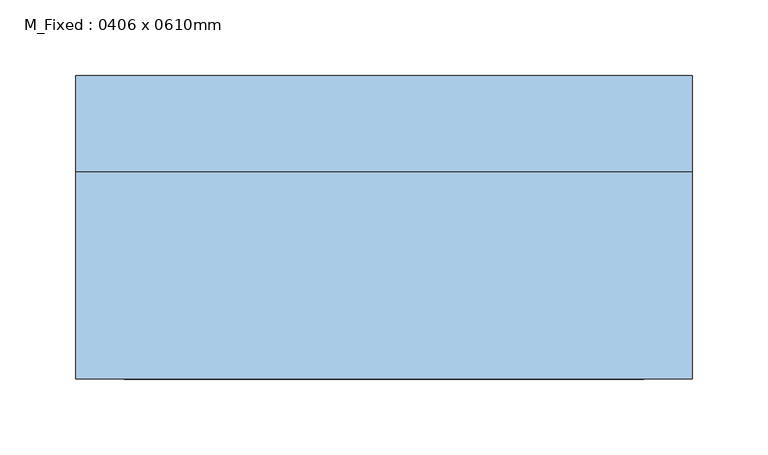
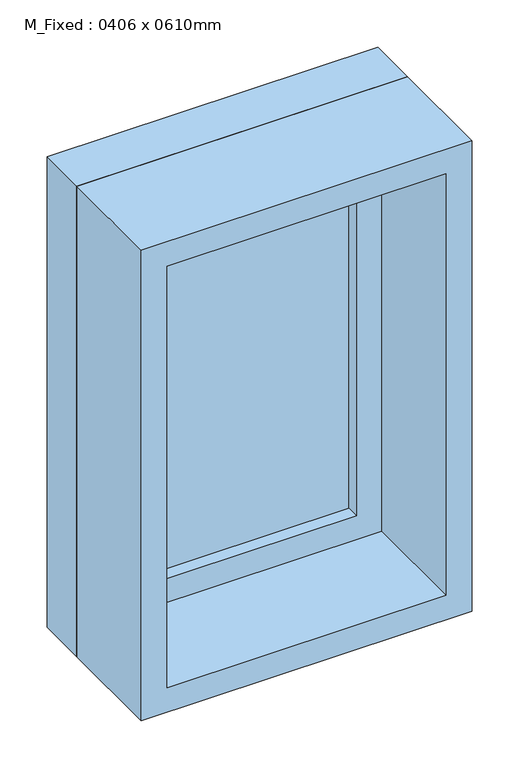
"""IFC4 building model written with IfcOpenShell, lengths in millimetres: window geometry, M_Fixed : 0406 x 0610mm."""

import ifcopenshell
import ifcopenshell.guid

model = None  # the IFC model being written
_history = None  # IfcOwnerHistory: only IFC2X3 demands one
_inside = {}  # id of a spatial element -> (the spatial element, [elements in it])
_under = {}  # id of a project, library or spatial element -> (it, [spatial elements below it])
_declared = {}  # id of a project -> (the project, [libraries it declares])
_typed = {}  # id of a type object -> (the type object, [elements of that type])
_made_of = {}  # id of a material, layer set ... -> (it, [elements and type objects made of it])


def new_model(schema):
    """Start an empty IFC model of exactly this schema.

    Asked for "IFC4X3", IfcOpenShell would pick the latest addendum, in which some entities
    have other attributes; the version numbers below select the first issue.
    IFC2X3 requires an IfcOwnerHistory on every rooted entity: one is made here for all.
    """
    global model, _history
    if schema == "IFC4X3":
        model = ifcopenshell.file(schema_version=(4, 3, 0, 0))
    else:
        model = ifcopenshell.file(schema=schema)
    _inside.clear()
    _under.clear()
    _declared.clear()
    _typed.clear()
    _made_of.clear()
    _history = None
    if model.schema == "IFC2X3":
        org = make("IfcOrganization", Name="unknown")
        user = make(
            "IfcPersonAndOrganization",
            ThePerson=make("IfcPerson", FamilyName="unknown"),
            TheOrganization=org,
        )
        app = make(
            "IfcApplication",
            ApplicationDeveloper=org,
            Version="unknown",
            ApplicationFullName="unknown",
            ApplicationIdentifier="unknown",
        )
        _history = make(
            "IfcOwnerHistory",
            OwningUser=user,
            OwningApplication=app,
            ChangeAction="ADDED",
            CreationDate=0,
        )
    return model


def make(cls, **values):
    """One entity of the class cls with the attributes given. An attribute that is None is left unset."""
    return model.create_entity(
        cls, **{name: value for name, value in values.items() if value is not None}
    )


def rooted(cls, **values):
    """An entity with a GlobalId (a new one), such as an element, a storey or a relation."""
    return make(cls, GlobalId=ifcopenshell.guid.new(), OwnerHistory=_history, **values)


def si_unit(unit_type, name, prefix=None):
    """IfcSIUnit, for example si_unit("LENGTHUNIT", "METRE", prefix="MILLI")."""
    return make("IfcSIUnit", UnitType=unit_type, Prefix=prefix, Name=name)


def assignment(units):
    """IfcUnitAssignment: the units of a project."""
    return None if units is None else make("IfcUnitAssignment", Units=units)


def point(xyz):
    """IfcCartesianPoint."""
    return None if xyz is None else make("IfcCartesianPoint", Coordinates=xyz)


def direction(xyz):
    """IfcDirection."""
    return None if xyz is None else make("IfcDirection", DirectionRatios=xyz)


def frame(location, z_axis=None, x_axis=None):
    """IfcAxis2Placement3D, a coordinate frame: its origin and axes. An axis left out is left unset."""
    return make(
        "IfcAxis2Placement3D",
        Location=point(location),
        Axis=direction(z_axis),
        RefDirection=direction(x_axis),
    )


def origin():
    """The frame at (0, 0, 0) with its axes left unset."""
    return frame((0.0, 0.0, 0.0))


def place(relative_to, where):
    """IfcLocalPlacement: puts the frame where relative to a parent placement (None: the world)."""
    return make(
        "IfcLocalPlacement", PlacementRelTo=relative_to, RelativePlacement=where
    )


def context(
    kind, dimensions, precision=None, world=None, true_north=None, identifier=None
):
    """IfcGeometricRepresentationContext, for example the 3D "Model" context."""
    return make(
        "IfcGeometricRepresentationContext",
        ContextIdentifier=identifier,
        ContextType=kind,
        CoordinateSpaceDimension=dimensions,
        Precision=precision,
        WorldCoordinateSystem=world,
        TrueNorth=true_north,
    )


def project(units=None, contexts=None):
    """IfcProject with its units and contexts."""
    return rooted(
        "IfcProject",
        Name="project",
        RepresentationContexts=contexts,
        UnitsInContext=assignment(units),
    )


def spatial(cls, under=None, at=None, **own):
    """A site, building, storey or space (cls), placed at a placement, below another one or the project."""
    s = rooted(cls, ObjectPlacement=at, **own)
    if under is not None:
        _under.setdefault(under.id(), (under, []))[1].append(s)
    return s


def polyline(points):
    """IfcPolyline through the points."""
    return make("IfcPolyline", Points=[point(p) for p in points])


def outline(outer, holes=None, kind="AREA"):
    """IfcArbitraryClosedProfileDef: a profile drawn as a closed curve; with holes, ...WithVoids."""
    if holes is None:
        return make("IfcArbitraryClosedProfileDef", ProfileType=kind, OuterCurve=outer)
    return make(
        "IfcArbitraryProfileDefWithVoids",
        ProfileType=kind,
        OuterCurve=outer,
        InnerCurves=holes,
    )


def extrude(swept, where, along, depth):
    """IfcExtrudedAreaSolid: the profile swept, set in the frame where, extruded along a direction by depth."""
    return make(
        "IfcExtrudedAreaSolid",
        SweptArea=swept,
        Position=where,
        ExtrudedDirection=direction(along),
        Depth=depth,
    )


def shape(context_of_items, identifier, shape_type, items):
    """IfcShapeRepresentation: the items that make up one representation, for example the "Body"."""
    return make(
        "IfcShapeRepresentation",
        ContextOfItems=context_of_items,
        RepresentationIdentifier=identifier,
        RepresentationType=shape_type,
        Items=items,
    )


def source(mapping_origin, context_of_items, identifier, shape_type, items):
    """IfcRepresentationMap: a shape defined once, which mapped items show again and again."""
    return make(
        "IfcRepresentationMap",
        MappingOrigin=mapping_origin,
        MappedRepresentation=shape(context_of_items, identifier, shape_type, items),
    )


def transform(
    local_origin,
    x_axis=None,
    y_axis=None,
    z_axis=None,
    scale=None,
    scale2=None,
    scale3=None,
    uniform=True,
):
    """IfcCartesianTransformationOperator3D, or its non-uniform kind. x_axis, y_axis, z_axis: its Axis1, 2, 3."""
    if uniform:
        return make(
            "IfcCartesianTransformationOperator3D",
            Axis1=direction(x_axis),
            Axis2=direction(y_axis),
            LocalOrigin=point(local_origin),
            Scale=scale,
            Axis3=direction(z_axis),
        )
    return make(
        "IfcCartesianTransformationOperator3DnonUniform",
        Axis1=direction(x_axis),
        Axis2=direction(y_axis),
        LocalOrigin=point(local_origin),
        Scale=scale,
        Axis3=direction(z_axis),
        Scale2=scale2,
        Scale3=scale3,
    )


def mapped(mapping_source, mapping_target):
    """IfcMappedItem: shows the shape of a source again, moved by a transform."""
    return make(
        "IfcMappedItem", MappingSource=mapping_source, MappingTarget=mapping_target
    )


def made_of(thing, what):
    """Note that an element or type object is made of a material, layer set ...; save() writes the relation."""
    if what is not None:
        _made_of.setdefault(what.id(), (what, []))[1].append(thing)
    return thing


def element(
    cls,
    number,
    at=None,
    inside=None,
    cuts=None,
    type_object=None,
    material=None,
    context=None,
    identifier="Body",
    shape_type=None,
    held_by="IfcProductDefinitionShape",
    body=None,
    shapes=None,
    **own,
):
    """One element of the class cls, such as IfcWall. Its Tag is "e" and its number.

    at: its placement. inside: the storey or other place that contains it. cuts: it is an
    opening in that element (IfcRelVoidsElement). A single representation is given by context,
    identifier, shape_type and body (its items); several are given by shapes. held_by: the class
    of the entity that holds the representations. save() writes the other relations.
    """
    e = rooted(cls, Tag="e%d" % number, ObjectPlacement=at, **own)
    if body is not None:
        shapes = [shape(context, identifier, shape_type, body)]
    if shapes is not None:
        e.Representation = make(held_by, Representations=shapes)
    if inside is not None:
        _inside.setdefault(inside.id(), (inside, []))[1].append(e)
    if cuts is not None:
        rooted(
            "IfcRelVoidsElement", RelatingBuildingElement=cuts, RelatedOpeningElement=e
        )
    if type_object is not None:
        _typed.setdefault(type_object.id(), (type_object, []))[1].append(e)
    return made_of(e, material)


def aggregate(whole, parts):
    """IfcRelAggregates: a whole, such as a stair, and the parts it consists of."""
    return rooted("IfcRelAggregates", RelatingObject=whole, RelatedObjects=parts)


def save(model, path):
    """Write the relations noted so far, then the file.

    IfcRelAggregates (storeys below a building ...), IfcRelContainedInSpatialStructure (elements
    in a storey), IfcRelDefinesByType, IfcRelAssociatesMaterial and IfcRelDeclares: one each for
    every whole, place, type object, material and project.
    """
    for whole, parts in _under.values():
        aggregate(whole, parts)
    for where, things in _inside.values():
        rooted(
            "IfcRelContainedInSpatialStructure",
            RelatedElements=things,
            RelatingStructure=where,
        )
    for kind, things in _typed.values():
        rooted("IfcRelDefinesByType", RelatedObjects=things, RelatingType=kind)
    for what, things in _made_of.values():
        rooted("IfcRelAssociatesMaterial", RelatedObjects=things, RelatingMaterial=what)
    for by, libraries in _declared.values():
        rooted("IfcRelDeclares", RelatingContext=by, RelatedDefinitions=libraries)
    model.write(path)


def m_fixed_0406_x_0610mm_8205b201(model_context):
    return source(origin(), model_context, "Body", "SweptSolid", [
        extrude(outline(polyline([(-140.0, 78.0), (140.0, 78.0), (140.0, 66.0), (-140.0, 66.0), (-140.0, 78.0)])), frame((0.0, 0.0, 978.0), z_axis=(0.0, 0.0, 1.0), x_axis=(1.0, 0.0, 0.0)), (0.0, 0.0, 1.0), 484.0),
        extrude(outline(polyline([(1506.0, -184.0), (934.0, -184.0), (934.0, 184.0), (1506.0, 184.0), (1506.0, -184.0)]), holes=[polyline([(1462.0, -140.0), (1462.0, 140.0), (978.0, 140.0), (978.0, -140.0), (1462.0, -140.0)])]), frame((0.0, 50.0, 0.0), z_axis=(0.0, 1.0, 0.0), x_axis=(0.0, 0.0, 1.0)), (0.0, 0.0, 1.0), 44.0),
        extrude(outline(polyline([(1525.0, -203.0), (915.0, -203.0), (915.0, 203.0), (1525.0, 203.0), (1525.0, -203.0)]), holes=[polyline([(1506.0, -184.0), (1506.0, 184.0), (934.0, 184.0), (934.0, -184.0), (1506.0, -184.0)])]), frame((0.0, 50.0, 0.0), z_axis=(0.0, 1.0, 0.0), x_axis=(0.0, 0.0, 1.0)), (0.0, 0.0, 1.0), 63.0),
        extrude(outline(polyline([(1525.0, -203.0), (915.0, -203.0), (915.0, 203.0), (1525.0, 203.0), (1525.0, -203.0)]), holes=[polyline([(1493.0, -171.0), (1493.0, 171.0), (947.0, 171.0), (947.0, -171.0), (1493.0, -171.0)])]), frame((0.0, -87.0, 0.0), z_axis=(0.0, 1.0, 0.0), x_axis=(0.0, 0.0, 1.0)), (0.0, 0.0, 1.0), 137.0),
    ])


if __name__ == "__main__":
    model = new_model("IFC4")
    model_context = context("Model", 3, world=origin())
    ifc_project = project(units=[si_unit("LENGTHUNIT", "METRE", prefix="MILLI")], contexts=[model_context])
    site = spatial("IfcSite", under=ifc_project)
    building = spatial("IfcBuilding", under=site)
    placement = place(None, origin())
    m_fixed_0406_x_0610mm_shape = m_fixed_0406_x_0610mm_8205b201(model_context)
    element("IfcWindow", 1, ObjectType="M_Fixed : 0406 x 0610mm", at=placement, inside=building, context=model_context, shape_type="MappedRepresentation", body=[
        mapped(m_fixed_0406_x_0610mm_shape, transform((0.0, 0.0, 0.0), x_axis=(1.0, 0.0, 0.0), y_axis=(0.0, 1.0, 0.0), z_axis=(0.0, 0.0, 1.0))),
    ])
    save(model, "model.ifc")

# Revit data of these elements
# Type "M_Fixed : 0406 x 0610mm"
#   Type Mark = "24"
#   Construction Type Id = "GSP4R"
#   Analytic Construction = "1/8 in Pilkington single glazing"
#   Visual Light Transmittance = 0.9
#   Thermal Resistance (R) = 0.271106 (m²·K)/W
#   Solar Heat Gain Coefficient = 0.78
#   Heat Transfer Coefficient (U) = 3.6886 W/(m²·K)
#   Height = 2' - 0.01575"
#   Default Sill Height = 3' - 0.02362"
#   Width = 1' - 3.98425"
#   Window Inset = 0' - 0.74803"
#   Frame Exterior Material = Sash
#   Frame Interior Material = Sash
#   Glass Pane Material = Glass
#   Sash = Sash
#   Wall Closure = (empty or 0)
# Element 1 (IfcWindow, "M_Fixed : 0406 x 0610mm")
#   Materials on its faces: "Sash", "Glass"
# Materials
#   "Sash": class "Wood", colour RGB 224 178 126, transparency 0, Cost = 0
#   "Glass": class "Glass", colour RGB 0 128 192, transparency 0.75, Description = "Soda Lime Glass", Cost = 0
